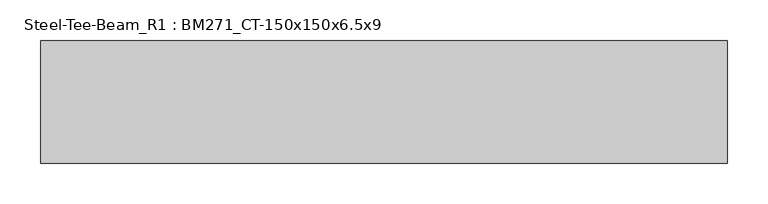
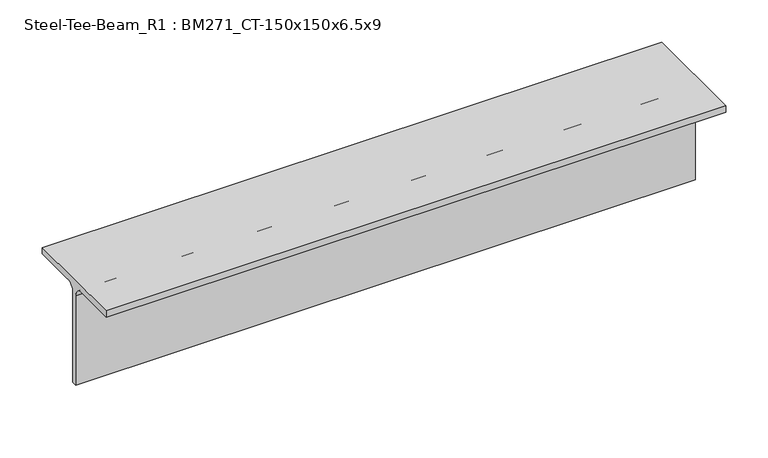
"""IFC4 building model written with IfcOpenShell, lengths in millimetres: member geometry, Steel-Tee-Beam_R1 : BM271_CT-150x150x6.5x9."""

from ifc_helpers import new_model, si_unit, point, frame, frame_2d, origin, place, context, project, spatial, polyline, circle_curve, trimmed, segment, composite_curve, outline, extrude, source, transform, mapped, element, save


def steel_tee_beam_r1_bm271_ct_150x150x6_5x9_96d46c3c(model_context):
    return source(origin(), model_context, "Body", "SweptSolid", [
        extrude(outline(composite_curve([segment(polyline([(-75.0, 75.0), (75.0, 75.0), (75.0, 66.0), (16.25, 66.0)]), True, "CONTINUOUS"), segment(trimmed(circle_curve(frame_2d((16.25, 53.0)), 13.0), [point((16.25, 66.0))], [point((3.25, 53.0))], True, "CARTESIAN"), True, "CONTINUOUS"), segment(polyline([(3.25, 53.0), (3.25, -75.0), (-3.25, -75.0), (-3.25, 53.0)]), True, "CONTINUOUS"), segment(trimmed(circle_curve(frame_2d((-16.25, 53.0)), 13.0), [point((-3.25, 53.0))], [point((-16.25, 66.0))], True, "CARTESIAN"), True, "CONTINUOUS"), segment(polyline([(-16.25, 66.0), (-75.0, 66.0), (-75.0, 75.0)]), True, "CONTINUOUS")], self_intersect=False)), frame((-500.0, 0.0, 0.0), z_axis=(1.0, 0.0, 0.0), x_axis=(0.0, 1.0, 0.0)), (0.0, 0.0, 1.0), 841.5608007),
    ])


if __name__ == "__main__":
    model = new_model("IFC4")
    model_context = context("Model", 3, world=origin())
    ifc_project = project(units=[si_unit("LENGTHUNIT", "METRE", prefix="MILLI")], contexts=[model_context])
    site = spatial("IfcSite", under=ifc_project)
    building = spatial("IfcBuilding", under=site)
    placement = place(None, origin())
    steel_tee_beam_r1_bm271_ct_150x150x6_5x9_shape = steel_tee_beam_r1_bm271_ct_150x150x6_5x9_96d46c3c(model_context)
    element("IfcMember", 1, ObjectType="Steel-Tee-Beam_R1 : BM271_CT-150x150x6.5x9", at=placement, inside=building, context=model_context, shape_type="MappedRepresentation", body=[
        mapped(steel_tee_beam_r1_bm271_ct_150x150x6_5x9_shape, transform((0.0, 0.0, 0.0), x_axis=(1.0, 0.0, 0.0), y_axis=(0.0, 1.0, 0.0), z_axis=(0.0, 0.0, 1.0))),
    ])
    save(model, "model.ifc")

# Revit data of these elements
# Type "Steel-Tee-Beam_R1 : BM271_CT-150x150x6.5x9"
#   Keynote = "CT-150x150x6.5x9"
#   Surface Area = 0.588841 m²/m
#   Section Area = 23.3904 cm²
#   Mass per Unit Length = 18.3614 kg/m
#   Length [instance default] = 1.5240 m
#   bf = 0.1500 m
#   d = 0.1500 m
#   k = 0.0220 m
#   r = 0.0130 m
#   tf = 0.0090 m
#   tw = 0.0065 m
#   hec_material4 [instance default] = none
#   hec_material3 [instance default] = none
#   hec_material2 [instance default] = none
#   hec_material1 [instance default] = none
#   Structural Material [instance default] = Steel, 45-345
#   Assembly Code = ""
# Element 1 (IfcMember, "Steel-Tee-Beam_R1 : BM271_CT-150x150x6.5x9")
#   Structural Material = none
# Materials
#   "Steel, 45-345": class "Metal", colour RGB 189 187 185, transparency 0, Description = "Steel 345 MPa", Cost = 0
